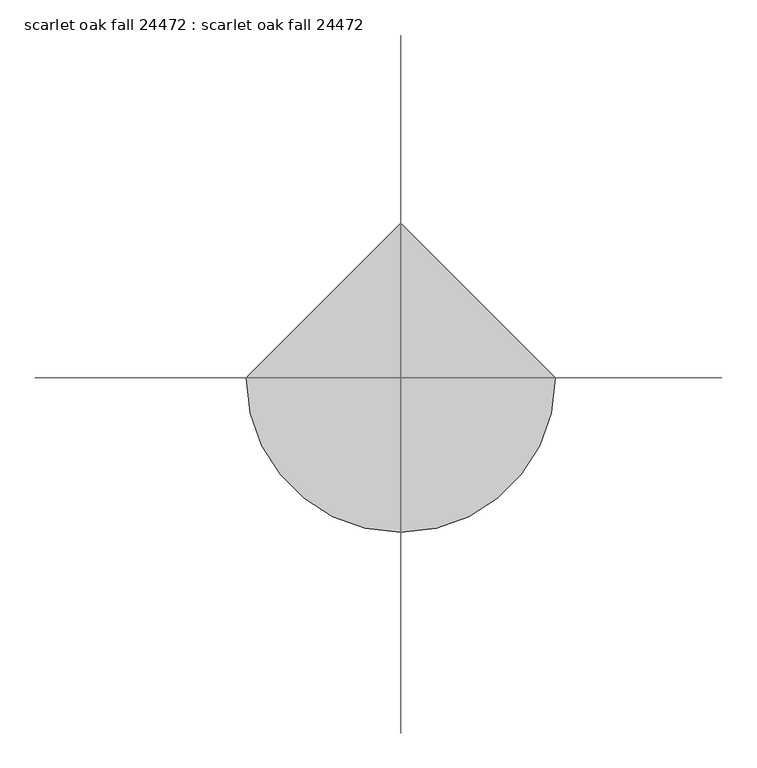
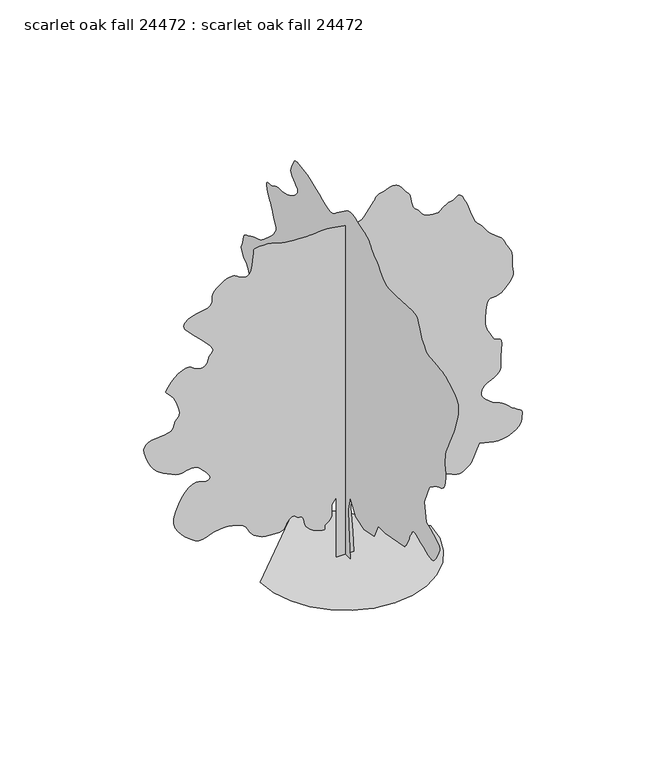
"""IFC4 building model written with IfcOpenShell, lengths in millimetres: proxy geometry, scarlet oak fall 24472 : scarlet oak fall 24472."""

from ifc_helpers import new_model, si_unit, origin, place, context, project, spatial, triangles, source, transform, mapped, element, save


def scarlet_oak_fall_24472_scarlet_oak_fall_24472_7ddbc09d(model_context):
    return source(origin(), model_context, "Body", "Tessellation", [
        triangles([(0.0175265, 310.9036245, 0.0), (0.0175265, -298.2620451, 0.0), (0.0175265, -200.0097575, 1159.3779247), (0.0175265, -180.3587949, 1709.5902706), (0.0175265, -298.2620451, 2220.5035618), (0.0175265, -612.6708881, 1709.5902706), (0.0175265, -1123.5817085, 1552.3870754), (0.0175265, -1713.0954346, 1689.9407433), (0.0175265, -1948.9013901, 2181.2021816), (0.0175265, -2361.5625389, 2181.2021816), (0.0175265, -3501.2886108, 2397.3587551), (0.0175265, -3543.2238419, 2447.9453476), (0.0175265, -3584.1434372, 2498.8747971), (0.0175265, -3622.9800201, 2550.4902512), (0.0175265, -3658.7176643, 2603.1445953), (0.0175265, -3690.3407341, 2657.1703674), (0.0175265, -3716.8074326, 2712.9233597), (0.0175265, -3737.102124, 2770.7082047), (0.0175265, -3756.8125488, 2830.2458496), (0.0175265, -3781.6790543, 2890.7994209), (0.0175265, -3810.8383209, 2952.2166023), (0.0175265, -3843.4264481, 3014.3197884), (0.0175265, -3878.6054054, 3076.9307922), (0.0175265, -3915.4862938, 3139.8972977), (0.0175265, -3953.2560814, 3203.0164101), (0.0175265, -3971.239286, 3223.4125488), (0.0175265, -3996.1057915, 3239.8717186), (0.0175265, -4034.7139, 3248.4060814), (0.0175265, -4093.9466217, 3245.0786682), (0.0175265, -4180.6878387, 3225.9525101), (0.0175265, -4301.7949814, 3187.039769), (0.0175265, -4464.1516411, 3124.4287651), (0.0175265, -4635.5763519, 3050.7434372), (0.0175265, -4781.5502907, 2984.9826256), (0.0175265, -4905.5273163, 2932.6079155), (0.0175265, -5010.9377426, 2899.1561783), (0.0175265, -5101.2345566, 2890.113707), (0.0175265, -5179.8222015, 2910.9670853), (0.0175265, -5250.1801163, 2967.228186), (0.0175265, -5321.172876, 3055.8486488), (0.0175265, -5394.553862, 3163.7225876), (0.0175265, -5463.1339783, 3281.2229736), (0.0175265, -5519.6741318, 3398.7233597), (0.0175265, -5556.9613907, 3506.5970078), (0.0175265, -5567.8072403, 3595.2430504), (0.0175265, -5544.9470078, 3654.9838806), (0.0175265, -5489.0922775, 3699.9671814), (0.0175265, -5408.4727798, 3750.0815643), (0.0175265, -5307.2539581, 3804.513707), (0.0175265, -5189.4995178, 3862.3750008), (0.0175265, -5059.4004822, 3922.8268341), (0.0175265, -4921.0467178, 3984.9805984), (0.0175265, -4778.5783791, 4047.9982635), (0.0175265, -4660.6716225, 4716.1196915), (0.0175265, -4955.4132248, 5403.875386), (0.0175265, -4964.7097504, 5417.0071426), (0.0175265, -4979.1367767, 5433.0346527), (0.0175265, -5003.9015442, 5454.9298279), (0.0175265, -5044.1101364, 5485.5872589), (0.0175265, -5104.9430511, 5527.903862), (0.0175265, -5191.5825302, 5584.850386), (0.0175265, -5309.1334946, 5659.3487457), (0.0175265, -5436.6669891, 5726.8364868), (0.0175265, -5549.7478775, 5770.9308884), (0.0175265, -5648.4011581, 5806.7955597), (0.0175265, -5732.6279938, 5849.5441132), (0.0175265, -5802.4016418, 5914.2884171), (0.0175265, -5857.7482635, 6016.1426651), (0.0175265, -5898.6422791, 6170.2443054), (0.0175265, -5922.3152527, 6321.6030899), (0.0175265, -5929.1223953, 6418.6564682), (0.0175265, -5923.915155, 6481.6735519), (0.0175265, -5911.4694031, 6530.949614), (0.0175265, -5896.6354248, 6586.7537659), (0.0175265, -5884.2152527, 6669.354538), (0.0175265, -5879.0080124, 6799.0722015), (0.0175265, -5880.8369705, 6942.175676), (0.0175265, -5888.8632248, 7060.8701752), (0.0175265, -5906.8464294, 7169.2769302), (0.0175265, -5938.5712372, 7281.4433395), (0.0175265, -5987.8467178, 7411.4917969), (0.0175265, -6058.4336884, 7573.5179535), (0.0175265, -6154.0900589, 7781.5947876), (0.0175265, -6244.9205612, 7969.6821442), (0.0175265, -6305.4738419, 8083.1694031), (0.0175265, -6346.419017, 8153.3494217), (0.0175265, -6378.4484573, 8211.4900589), (0.0175265, -6412.2045364, 8288.8835907), (0.0175265, -6458.3057922, 8416.8234558), (0.0175265, -6527.4701752, 8626.5513519), (0.0175265, -6601.9935333, 8869.1720078), (0.0175265, -6652.1329147, 9078.1127426), (0.0175265, -6670.2940155, 9258.1732635), (0.0175265, -6648.9075302, 9414.1800201), (0.0175265, -6580.4541504, 9550.9338821), (0.0175265, -6457.3407349, 9673.2345566), (0.0175265, -6271.9968155, 9785.9340729), (0.0175265, -6092.164769, 9878.5679535), (0.0175265, -5973.8772217, 9942.3477814), (0.0175265, -5892.0130325, 9984.43591), (0.0175265, -5821.4772217, 10012.1214294), (0.0175265, -5737.1998077, 10032.5690186), (0.0175265, -5614.0858109, 10053.0154449), (0.0175265, -5427.0402512, 10080.7009644), (0.0175265, -5226.405986, 10102.5205627), (0.0175265, -5070.8056, 10110.9526062), (0.0175265, -4947.513707, 10121.4182465), (0.0175265, -4843.8310822, 10149.4339783), (0.0175265, -4747.0061783, 10210.4442078), (0.0175265, -4644.3394798, 10319.9445007), (0.0175265, -4523.1050194, 10493.3501953), (0.0175265, -4417.2379349, 10684.0025116), (0.0175265, -4354.6778, 10837.2152527), (0.0175265, -4313.7837845, 10956.3661194), (0.0175265, -4272.8641891, 11044.9362946), (0.0175265, -4210.3040543, 11106.353476), (0.0175265, -4104.4369698, 11144.0476868), (0.0175265, -3933.5965256, 11161.4710419), (0.0175265, -2990.3674713, 11102.5176636), (0.0175265, -2816.5045372, 11105.5663147), (0.0175265, -2674.9503868, 11105.1593628), (0.0175265, -2554.6812744, 11112.322879), (0.0175265, -2444.7449615, 11138.027124), (0.0175265, -2334.1178478, 11193.3225861), (0.0175265, -2211.8040928, 11289.1574341), (0.0175265, -2066.8032051, 11436.5786682), (0.0175265, -1927.0752514, 11585.474231), (0.0175265, -1822.4043148, 11686.9215271), (0.0175265, -1744.5483112, 11753.6721039), (0.0175265, -1685.2519306, 11798.4275116), (0.0175265, -1636.2706181, 11833.8858124), (0.0175265, -1589.3492088, 11872.7729736), (0.0175265, -1536.2428574, 11927.8405426), (0.0175265, -1485.2548359, 11992.8644806), (0.0175265, -1443.5456085, 12053.4177612), (0.0175265, -1401.1529926, 12109.8573395), (0.0175265, -1348.1024517, 12162.4855225), (0.0175265, -1274.4272976, 12211.7104248), (0.0175265, -1170.1577173, 12257.8366791), (0.0175265, -1025.3294209, 12301.1944977), (0.0175265, -862.7415253, 12348.971814), (0.0175265, -711.1517956, 12401.9057922), (0.0175265, -569.5289721, 12450.7249054), (0.0175265, -436.8469909, 12486.1320465), (0.0175265, -312.0695054, 12498.8580139), (0.0175265, -194.1657283, 12479.604538), (0.0175265, -82.1065163, 12419.1012543), (0.0175265, 507.4081999, 11986.7939209), (0.0175265, 571.2282506, 11928.7044434), (0.0175265, 632.9883253, 11875.7704651), (0.0175265, 700.2449759, 11833.124231), (0.0175265, 780.5673986, 11805.9712372), (0.0175265, 881.5121092, 11799.4437286), (0.0175265, 1010.6431807, 11818.6960419), (0.0175265, 1175.5247589, 11868.8871643), (0.0175265, 1362.6338322, 11943.4105225), (0.0175265, 1551.1170948, 12027.2309875), (0.0175265, 1737.537838, 12112.7780914), (0.0175265, 1918.4594982, 12192.4581116), (0.0175265, 2090.445512, 12258.7517395), (0.0175265, 2250.0539383, 12304.0652527), (0.0175265, 2393.8535912, 12320.8549255), (0.0175265, 2524.6458984, 12330.0241333), (0.0175265, 2646.1466217, 12350.8775116), (0.0175265, 2756.3317566, 12373.4331116), (0.0175265, 2853.0805023, 12387.7578186), (0.0175265, 2934.3860046, 12383.8720093), (0.0175265, 2998.139962, 12351.7914093), (0.0175265, 3042.3105217, 12281.5352325), (0.0175265, 3081.7819496, 12193.2708527), (0.0175265, 3127.0957535, 12111.863031), (0.0175265, 3169.6661201, 12034.5712372), (0.0175265, 3200.9081085, 11958.6502899), (0.0175265, 3212.1856178, 11881.3840759), (0.0175265, 3194.9389961, 11799.9762543), (0.0175265, 3140.5830116, 11711.6862946), (0.0175265, 3057.3979729, 11630.7877441), (0.0175265, 2968.3455597, 11567.4148682), (0.0175265, 2886.8880318, 11512.6519318), (0.0175265, 2826.3850388, 11457.5343658), (0.0175265, 2800.2738419, 11393.1452728), (0.0175265, 2821.9146721, 11310.5445007), (0.0175265, 2904.7694984, 11200.765155), (0.0175265, 3019.1712364, 11091.3927612), (0.0175265, 3127.0448845, 11011.6115845), (0.0175265, 3229.076738, 10954.8173767), (0.0175265, 3325.9522202, 10914.5582062), (0.0175265, 3418.3576263, 10884.2309875), (0.0175265, 3507.0033783, 10857.3826263), (0.0175265, 3592.525193, 10827.4112), (0.0175265, 3677.9455605, 10804.3219116), (0.0175265, 3765.7785713, 10796.7026093), (0.0175265, 3855.9995178, 10795.9654449), (0.0175265, 3948.6333984, 10793.5016418), (0.0175265, 4043.6802132, 10780.7256775), (0.0175265, 4141.139962, 10749.0264496), (0.0175265, 4240.9873558, 10689.8695953), (0.0175265, 4344.1874519, 10637.3169891), (0.0175265, 4445.6350388, 10618.4704651), (0.0175265, 4536.4402519, 10614.0509674), (0.0175265, 4607.6617767, 10604.8306), (0.0175265, 4650.3338814, 10571.5570496), (0.0175265, 4655.540831, 10494.9500977), (0.0175265, 4614.3674721, 10355.8085907), (0.0175265, 4553.5089775, 10209.3779938), (0.0175265, 4502.988224, 10110.7247131), (0.0175265, 4458.6400589, 10040.2394806), (0.0175265, 4416.3743248, 9978.3653503), (0.0175265, 4372.025869, 9905.4918915), (0.0175265, 4321.4798264, 9802.0377411), (0.0175265, 4260.6469116, 9648.393631), (0.0175265, 4196.3595566, 9497.2633209), (0.0175265, 4141.038224, 9401.8104263), (0.0175265, 4098.7472008, 9343.1361008), (0.0175265, 4073.6522209, 9302.3438232), (0.0175265, 4069.8675682, 9260.5353287), (0.0175265, 4091.5336876, 9198.7629364), (0.0175265, 4142.740155, 9098.1789597), (0.0175265, 4233.9008698, 8964.8539581), (0.0175265, 4361.815155, 8823.2998077), (0.0175265, 4510.3796333, 8682.0758698), (0.0175265, 4663.3894798, 8549.7926651), (0.0175265, 4804.7404449, 8435.0357162), (0.0175265, 4918.2277039, 8346.4149628), (0.0175265, 4987.7217178, 8292.4909286), (0.0175265, 5049.4185333, 8258.7592667), (0.0175265, 5142.0524139, 8224.6723938), (0.0175265, 5253.2537659, 8189.9000977), (0.0175265, 5370.6524139, 8154.0860046), (0.0175265, 5481.8537659, 8116.9004837), (0.0175265, 5574.4876465, 8078.0133224), (0.0175265, 5636.1838806, 8037.0425674), (0.0175265, 5687.8475876, 8003.0068542), (0.0175265, 5753.6336884, 7978.9530899), (0.0175265, 5825.9217178, 7955.5853302), (0.0175265, 5897.1941116, 7923.6064682), (0.0175265, 5959.8815643, 7873.7717194), (0.0175265, 6006.3891907, 7796.7589783), (0.0175265, 6029.1982635, 7683.3222977), (0.0175265, 6047.8674728, 7569.3780899), (0.0175265, 6079.9474915, 7488.7835907), (0.0175265, 6114.7709473, 7429.1447891), (0.0175265, 6141.7204651, 7378.0903473), (0.0175265, 6150.0769318, 7323.2774139), (0.0175265, 6129.2235535, 7252.2846542), (0.0175265, 6068.4917953, 7152.7674728), (0.0175265, 5993.1045364, 7059.5493256), (0.0175265, 5932.1448853, 7003.8213318), (0.0175265, 5880.8113907, 6967.6776077), (0.0175265, 5834.2787659, 6933.2349426), (0.0175265, 5787.7711395, 6882.638031), (0.0175265, 5736.437645, 6798.030986), (0.0175265, 5675.4779938, 6661.5055984), (0.0175265, 5609.0314682, 6524.7523178), (0.0175265, 5548.0712357, 6438.5447891), (0.0175265, 5498.1097504, 6383.604538), (0.0175265, 5464.6577225, 6340.6786697), (0.0175265, 5453.2026077, 6290.5642868), (0.0175265, 5469.2295364, 6213.9579163), (0.0175265, 5518.277124, 6091.6566605), (0.0175265, 5583.4283798, 5957.8747101), (0.0175265, 5644.7694031, 5854.0141891), (0.0175265, 5703.392569, 5771.4645767), (0.0175265, 5760.2629349, 5701.6141891), (0.0175265, 5816.4734573, 5635.9048279), (0.0175265, 5873.0136108, 5565.7242279), (0.0175265, 5930.9257736, 5482.4886108), (0.0175265, 5998.1338806, 5400.3959473), (0.0175265, 6076.3407349, 5333.4157333), (0.0175265, 6157.2904449, 5272.6339783), (0.0175265, 6232.753862, 5209.0832062), (0.0175265, 6294.4506775, 5133.8738434), (0.0175265, 6334.1505798, 5038.0139969), (0.0175265, 6343.5994217, 4912.614093), (0.0175265, 6351.5495178, 4814.1384178), (0.0175265, 6380.8355209, 4781.651738), (0.0175265, 6414.2369705, 4780.1024139), (0.0175265, 6434.5822403, 4774.4382248), (0.0175265, 6424.6508698, 4729.5816605), (0.0175265, 6367.3229736, 4610.4810814), (0.0175265, 6245.3519302, 4382.0589775), (0.0175265, 6117.819017, 4125.8490349), (0.0175265, 6040.8312744, 3937.3811783), (0.0175265, 5992.6981659, 3802.5071434), (0.0175265, 5951.8041504, 3707.1809853), (0.0175265, 5896.4575287, 3637.2800194), (0.0175265, 5805.0177612, 3578.7330116), (0.0175265, 5655.8437271, 3517.4428574), (0.0175265, 5483.6059845, 3467.7098465), (0.0175265, 5332.0187256, 3446.8561775), (0.0175265, 5192.8016418, 3445.2559845), (0.0175265, 5057.7244217, 3453.2825294), (0.0175265, 4918.5067566, 3461.2834946), (0.0175265, 4766.9197884, 3459.6833015), (0.0175265, 4594.7076256, 3438.8299232), (0.0175265, 4422.952993, 3420.1610046), (0.0175265, 4274.5661201, 3424.1741318), (0.0175265, 4144.0610046, 3439.8714294), (0.0175265, 4025.9254829, 3456.2544411), (0.0175265, 3914.6735527, 3462.3250008), (0.0175265, 3804.7930504, 3447.0849426), (0.0175265, 3690.7723938, 3399.5361008), (0.0175265, 3581.6540543, 3348.9900581), (0.0175265, 3491.4078186, 3322.5233597), (0.0175265, 3422.1419884, 3305.6831085), (0.0175265, 3375.9139961, 3284.0422783), (0.0175265, 3354.7812744, 3243.1229736), (0.0175265, 3360.8009651, 3168.5484558), (0.0175265, 3396.0307915, 3045.815831), (0.0175265, 3452.8505791, 2915.4374519), (0.0175265, 3521.0243248, 2823.1846527), (0.0175265, 3598.6722015, 2762.7581085), (0.0175265, 3683.8638039, 2727.7567566), (0.0175265, 3774.7195953, 2711.8309845), (0.0175265, 3869.3600395, 2708.6053093), (0.0175265, 3965.8800201, 2711.7548264), (0.0175265, 4339.2598457, 2299.1064674), (0.0175265, 4368.5208504, 2252.6422977), (0.0175265, 4396.5877419, 2205.3220757), (0.0175265, 4422.2672791, 2156.2823364), (0.0175265, 4444.3144798, 2104.6617954), (0.0175265, 4461.5608109, 2049.6073071), (0.0175265, 4472.7877419, 1990.2551159), (0.0175265, 4476.800869, 1925.7468441), (0.0175265, 4476.115155, 1858.4875774), (0.0175265, 4471.314576, 1791.9167862), (0.0175265, 4458.2333977, 1726.7225098), (0.0175265, 4432.8082054, 1663.588282), (0.0175265, 4390.8726837, 1603.2049038), (0.0175265, 4328.3125488, 1546.2580891), (0.0175265, 4240.9873558, 1493.4361679), (0.0175265, 4157.7008698, 1448.5772781), (0.0175265, 4099.153862, 1413.687838), (0.0175265, 4049.1917953, 1386.7054733), (0.0175265, 3991.6610046, 1365.5650486), (0.0175265, 3910.4316605, 1348.2066605), (0.0175265, 3789.3245178, 1332.5653187), (0.0175265, 3612.1850395, 1316.5811199), (0.0175265, 3410.6865829, 1318.8721138), (0.0175265, 3225.0127419, 1354.1629829), (0.0175265, 3051.7084946, 1414.5488319), (0.0175265, 2887.3449806, 1492.1179344), (0.0175265, 2728.4933395, 1578.9707726), (0.0175265, 2571.6738419, 1667.1976547), (0.0175265, 2413.5029732, 1748.8916508), (0.0175265, 2272.4543152, 1823.1968536), (0.0175265, 2163.3739094, 1893.3770176), (0.0175265, 2077.3237839, 1957.7152416), (0.0175265, 2005.3681469, 2014.4892471), (0.0175265, 1938.5687359, 2061.9822784), (0.0175265, 1867.9871429, 2098.4769985), (0.0175265, 1784.687867, 2122.2512741), (0.0175265, 1693.0802319, 2142.3020851), (0.0175265, 1602.8492569, 2167.1661198), (0.0175265, 1512.9611389, 2194.438147), (0.0175265, 1422.387307, 2221.7075581), (0.0175265, 1330.0913418, 2246.5715927), (0.0175265, 1235.0471432, 2266.6224037), (0.0175265, 1136.2233061, 2279.4544693), (0.0175265, 1035.1643583, 2286.1575485), (0.0175265, 934.1027945, 2289.7669212), (0.0175265, 833.0438467, 2290.7981083), (0.0175265, 731.9848263, 2289.7669212), (0.0175265, 630.9258785, 2287.1887356), (0.0175265, 529.864351, 2283.5795082), (0.0175265, 428.8053669, 2279.4544693), (0.0175265, 232.3013002, 1984.6976063), (0.0175265, 192.9998656, 1532.7376934), (284.9321357, 0.0006104, 0.0093596), (-304.5815722, 0.0006104, 0.0093596), (-304.5815722, 0.0004832, 2161.5603573), (-461.7872563, 0.0004832, 1945.4063999), (-461.7872563, 0.0005087, 1709.6004444), (-458.17792, 0.0005087, 1654.888813), (-458.17792, 0.0005087, 1600.3473747), (-465.3965927, 0.0005087, 1546.1514095), (-483.4407675, 0.0005341, 1492.4709652), (-515.9248312, 0.0005341, 1439.4789963), (-566.4555768, 0.0005341, 1387.3429344), (-638.6398699, 0.0005341, 1336.2406757), (-695.1853283, 0.0005341, 1283.1902802), (-710.8266701, 0.0005341, 1229.4514091), (-707.2172974, 0.0005341, 1181.559783), (-706.0133738, 0.0005341, 1146.037896), (-728.8733156, 0.0005341, 1129.4237211), (-797.4482723, 0.0005341, 1138.2476738), (-933.3966602, 0.0005341, 1179.0375532), (-1088.4814528, 0.0005341, 1242.5731373), (-1204.3791023, 0.0005341, 1314.3561104), (-1287.6199516, 0.0005341, 1393.0172974), (-1344.7395756, 0.0005341, 1477.1750965), (-1382.2654827, 0.0005087, 1565.4579346), (-1406.7282337, 0.0005087, 1656.4914768), (-1424.6607147, 0.0005087, 1748.9018246), (-1429.2428478, 0.0005087, 1774.0502895), (-1436.0601643, 0.0005087, 1798.5130405), (-1447.3453766, 0.0005087, 1821.6042183), (-1465.3361389, 0.0005087, 1842.6277897), (-1492.2602222, 0.0005087, 1860.9031277), (-1530.3602222, 0.0005087, 1875.7417568), (-1581.8637646, 0.0005087, 1886.4554924), (-1633.3673069, 0.0005087, 1904.0983109), (-1673.8702126, 0.0005087, 1933.7757145), (-1709.219363, 0.0004832, 1965.8584946), (-1745.2543728, 0.0004832, 1990.7225292), (-1787.8222687, 0.0004832, 1998.7438419), (-1842.7623745, 0.0004832, 1980.2958401), (-1915.9220078, 0.0005087, 1925.7544018), (-1980.257761, 0.0005087, 1849.4451061), (-2016.7524811, 0.0005087, 1774.8530022), (-2043.2776062, 0.0005087, 1706.1053089), (-2077.707336, 0.0005087, 1647.3247398), (-2137.9206665, 0.0005087, 1602.6409847), (-2241.7862743, 0.0005087, 1576.1716702), (-2407.1834461, 0.0005087, 1572.0466312), (-2589.9363899, 0.0005087, 1584.1929829), (-2738.3232628, 0.0005087, 1604.2437939), (-2858.8464294, 0.0005087, 1632.8898651), (-2958.0839767, 0.0005087, 1670.8145851), (-3042.5389961, 0.0005087, 1718.7089001), (-3118.713707, 0.0005087, 1777.2608494), (-3193.211776, 0.0005087, 1847.1541122), (-3256.3817574, 0.0005087, 1923.8062649), (-3301.7205597, 0.0004832, 2000.8063614), (-3340.1507721, 0.0004832, 2076.0843246), (-3382.7214294, 0.0004832, 2147.5827221), (-3440.4048271, 0.0004832, 2213.2367088), (-3524.2247108, 0.0004832, 2270.9860909), (-3645.154248, 0.0004832, 2318.7660233), (-3766.7439194, 0.0004832, 2355.0854633), (-3854.9580116, 0.0004578, 2380.7522106), (-3924.6302124, 0.0004578, 2397.1378384), (-3990.5180511, 0.0004578, 2405.6162453), (-4067.3781853, 0.0004578, 2407.5645275), (-4170.0451744, 0.0004578, 2404.3564384), (-4313.275676, 0.0004578, 2397.3663128), (-4470.7555984, 0.0004578, 2372.5607048), (-4610.7351357, 0.0004832, 2326.4420082), (-4739.6909271, 0.0004832, 2276.1982727), (-4864.1763519, 0.0004832, 2239.0176933), (-4990.7447891, 0.0004832, 2232.0859943), (-5125.8725876, 0.0004832, 2272.5889), (-5276.1389969, 0.0004578, 2377.7169308), (-5433.3648651, 0.0004578, 2518.3058784), (-5578.5257721, 0.0004578, 2657.8560814), (-5702.0461395, 0.0004324, 2802.5853287), (-5794.2736496, 0.0004324, 2958.6429543), (-5845.6071442, 0.0004324, 3132.226545), (-5846.4198853, 0.0004069, 3329.5336876), (-5787.0601364, 0.0004069, 3556.7366798), (-5687.7208511, 0.0003815, 3785.8956573), (-5577.0276077, 0.0003815, 3982.4153481), (-5458.1046341, 0.0003561, 4142.4861008), (-5334.0255798, 0.0003561, 4262.3232628), (-5207.8635132, 0.0003561, 4338.1677612), (-5082.7432434, 0.0003561, 4366.2602325), (-4961.7378387, 0.0003561, 4342.765155), (-4847.6154442, 0.0003561, 4303.2428581), (-4746.5742279, 0.0003561, 4286.3770271), (-4666.8183403, 0.0003561, 4293.2606186), (-4616.6277992, 0.0003561, 4324.8833977), (-4604.2582054, 0.0003561, 4382.2874519), (-4637.9384171, 0.0003561, 4466.5139969), (-4725.9240349, 0.0003306, 4578.5786682), (-4828.540155, 0.0003306, 4690.9738426), (-4906.7470093, 0.0003306, 4777.5877419), (-4969.8146713, 0.0003306, 4841.5195953), (-5027.0414108, 0.0003306, 4885.8680511), (-5087.7220093, 0.0003306, 4913.7064682), (-5161.1024139, 0.0003052, 4928.1590744), (-5256.5047302, 0.0003052, 4932.2739395), (-5354.3458511, 0.0003306, 4923.0535721), (-5435.3717194, 0.0003306, 4901.7938232), (-5509.1584946, 0.0003306, 4878.1464294), (-5585.3584946, 0.0003306, 4861.6872597), (-5673.5728775, 0.0003306, 4862.0936302), (-5783.4533798, 0.0003306, 4888.9666992), (-5924.6261581, 0.0003052, 4951.9332047), (-6074.4356186, 0.0003052, 5027.2698853), (-6206.363031, 0.0003052, 5092.6240356), (-6324.2192093, 0.0003052, 5159.730986), (-6431.7376465, 0.0003052, 5240.2231659), (-6532.7529922, 0.0003052, 5345.7859085), (-6631.0004837, 0.0002798, 5488.1528), (-6730.2891907, 0.0002798, 5679.0085922), (-6812.3818542, 0.0002543, 5877.0523178), (-6857.6953674, 0.0002543, 6036.2594604), (-6867.9569504, 0.0002543, 6161.1006775), (-6844.8682434, 0.0002289, 6256.0204651), (-6790.157048, 0.0002289, 6325.5144791), (-6705.5494217, 0.0002289, 6374.0283783), (-6592.7225876, 0.0002289, 6406.0578186), (-6459.5249039, 0.0002289, 6424.4473938), (-6318.7834946, 0.0002289, 6435.2932434), (-6179.7187271, 0.0002289, 6447.8157349), (-6051.677124, 0.0002289, 6471.3613907), (-5943.9302124, 0.0002289, 6515.201738), (-5865.7239395, 0.0002289, 6588.5821426), (-5826.3536682, 0.0002035, 6700.8252914), (-5797.2705597, 0.0002035, 6809.207048), (-5752.3384186, 0.0002035, 6879.7934372), (-5704.6878387, 0.0002035, 6934.9115845), (-5667.3244217, 0.0002035, 6996.8874527), (-5653.3543442, 0.000178, 7088.0987457), (-5675.8082062, 0.000178, 7230.8720078), (-5747.7660233, 0.000178, 7447.5343643), (-5849.6708496, 0.0001526, 7660.9451752), (-5947.1305984, 0.0001526, 7795.2858124), (-6030.8237457, 0.0001526, 7874.990831), (-6091.5043442, 0.0001272, 7924.4192093), (-6119.8508698, 0.0001272, 7968.0055023), (-6106.6173752, 0.0001272, 8030.1848465), (-6042.5079163, 0.0001272, 8135.3156387), (-5939.1805023, 0.0001272, 8266.5064682), (-5819.6738434, 0.0001017, 8386.0137085), (-5691.911293, 0.0001017, 8486.9528961), (-5563.7941132, 0.0001017, 8562.4674728), (-5443.2712372, 0.0001017, 8605.6473953), (-5338.1910233, 0.0001017, 8609.6605225), (-5256.5047302, 0.0001017, 8567.6235535), (-5176.4183395, 0.0001017, 8504.9361008), (-5077.7650589, 0.0001017, 8456.015831), (-4970.8564682, 0.0001017, 8427.3646729), (-4866.0050194, 0.0001017, 8425.5357147), (-4773.5490349, 0.0001017, 8457.0570465), (-4703.7753868, 0.0001017, 8528.4311783), (-4666.9962364, 0.0001017, 8646.2111984), (-4633.2904449, 0.0001017, 8758.5043442), (-4580.3567574, 7.63e-05, 8825.0776062), (-4529.8360039, 7.63e-05, 8869.9853302), (-4503.3693054, 7.63e-05, 8917.3051163), (-4522.6224907, 7.63e-05, 8991.0924728), (-4609.2366806, 7.63e-05, 9115.425), (-4784.902993, 5.09e-05, 9314.3326263), (-5005.1718155, 5.09e-05, 9539.0212372), (-5202.0725876, 2.54e-05, 9728.3021255), (-5361.8639969, 2.54e-05, 9887.6871643), (-5470.753862, 2.54e-05, 10022.6626465), (-5515.0511581, 0.0, 10138.7404449), (-5480.9642853, 0.0, 10241.4074341), (-5354.7522217, 0.0, 10336.1493256), (-5186.4258682, 0.0, 10409.1483582), (-5035.6519318, 0.0, 10450.8562775), (-4903.089093, 0.0, 10473.3095581), (-4789.4242287, -2.54e-05, 10488.5493256), (-4695.3424713, -2.54e-05, 10508.5899628), (-4621.5554054, -2.54e-05, 10545.4958496), (-4568.7234558, -2.54e-05, 10611.2569519), (-4542.3837845, -2.54e-05, 10689.0568542), (-4538.3706573, -2.54e-05, 10757.2306), (-4542.9424713, -2.54e-05, 10820.603476), (-4542.3837845, -2.54e-05, 10883.9763519), (-4522.9018341, -5.09e-05, 10952.1500977), (-4470.7555984, -5.09e-05, 11029.95), (-4372.2290543, -5.09e-05, 11122.1780914), (-4251.6300201, -5.09e-05, 11213.4399628), (-4141.3431473, -5.09e-05, 11284.4333038), (-4039.6667953, -7.63e-05, 11334.0895752), (-3944.8487457, -7.63e-05, 11361.4204651), (-3855.1867767, -7.63e-05, 11365.3830139), (-3768.9536682, -7.63e-05, 11344.909845), (-3684.4733597, -5.09e-05, 11299.0382263), (-3597.3766411, -5.09e-05, 11242.9544403), (-3507.5623558, -5.09e-05, 11199.2408295), (-3419.4497108, -5.09e-05, 11177.8549255), (-3337.5093636, -5.09e-05, 11188.8019318), (-3266.2369698, -5.09e-05, 11242.0149628), (-3210.1028961, -7.63e-05, 11347.5015472), (-3173.5522202, -7.63e-05, 11515.1924744), (-3151.7337845, -7.63e-05, 11695.2524139), (-3136.0873558, -0.0001017, 11834.3939209), (-3125.5970078, -0.0001017, 11937.4666992), (-3119.2471046, -0.0001017, 12009.2472015), (-3115.9705605, -0.0001017, 12054.5607147), (-3114.776738, -0.0001017, 12078.2336884), (-3114.5988419, -0.0001017, 12085.0414124), (-3088.7669884, -0.0001017, 12089.0539581), (-3018.5869698, -0.0001017, 12097.8929535), (-2915.0563705, -0.0001017, 12106.7075317), (-2789.1995178, -0.0001017, 12110.7200775), (-2651.988707, -0.0001017, 12105.1064667), (-2514.4299522, -0.0001017, 12085.0414124), (-2387.5340641, -0.0001017, 12045.7472992), (-2271.1766315, -0.0001017, 12002.0336884), (-2154.476342, -0.0001017, 11970.3600403), (-2032.2769695, -0.0001017, 11948.286969), (-1899.419672, -0.0001017, 11933.4541534), (-1750.7534557, -0.0001017, 11923.4466248), (-1581.1170078, -0.0001017, 11915.8261597), (-1385.3567184, -0.0001017, 11908.2056946), (-1196.4162163, -0.0001017, 11907.1139008), (-1040.8158302, -0.0001017, 11916.3342682), (-903.7777559, -0.0001017, 11929.3392883), (-770.5217182, -0.0001017, 11939.6002899), (-626.2675146, -0.0001017, 11940.5653473), (-456.2297467, -0.0001017, 11925.7325317), (-245.6314641, -0.0001017, 11888.5464294), (-32.7413631, -0.0001017, 11844.3247101), (138.8999065, -0.0001017, 11813.8451752), (276.1665915, -0.0001017, 11798.8333008), (385.9352365, -0.0001017, 11800.9924713), (475.0790686, -0.0001017, 11822.1004852), (550.4713417, -0.0001017, 11863.8072418), (618.9904152, -0.0001017, 11927.8405426), (913.7472782, -0.0001272, 12301.1944977), (957.9762646, -0.0001272, 12358.7770294), (993.267061, -0.0001272, 12412.929538), (1025.1186052, -0.0001272, 12462.586972), (1059.035285, -0.0001272, 12506.7575317), (1100.5134218, -0.0001272, 12544.3994202), (1155.0548601, -0.0001272, 12574.4731659), (1228.1561394, -0.0001272, 12595.9625519), (1317.7570656, -0.0001526, 12620.5994202), (1415.6080696, -0.0001526, 12653.4927612), (1517.9269695, -0.0001526, 12683.6176666), (1620.9366703, -0.0001526, 12700.0003876), (1720.8500484, -0.0001526, 12691.6439209), (1813.8876835, -0.0001526, 12647.5245209), (1896.2726257, -0.0001272, 12556.6684387), (1969.4296429, -0.0001272, 12453.0363922), (2036.4018631, -0.0001272, 12372.4168945), (2095.8124809, -0.0001272, 12306.5802155), (2146.2848362, -0.0001272, 12247.2966248), (2186.4447395, -0.0001272, 12186.2852325), (2214.9181469, -0.0001017, 12115.2918915), (2230.3283981, -0.0001017, 12026.0880341), (2241.0421337, -0.0001017, 11933.6320496), (2255.8807629, -0.0001017, 11856.6437256), (2274.1561008, -0.0001017, 11792.534848), (2295.1796722, -7.63e-05, 11738.736969), (2318.2682339, -7.63e-05, 11692.6618744), (2342.7309849, -7.63e-05, 11651.7678589), (2367.882066, -7.63e-05, 11613.4388031), (2393.3175774, -7.63e-05, 11596.1921814), (2419.7868919, -7.63e-05, 11576.5329163), (2448.3162552, -7.63e-05, 11552.0727814), (2479.9416504, -7.63e-05, 11520.3991333), (2515.6897591, -7.63e-05, 11479.0981659), (2556.5863907, -7.63e-05, 11425.7583984), (2603.677993, -7.63e-05, 11357.9916046), (2673.4772209, -5.09e-05, 11293.5769318), (2772.1307922, -5.09e-05, 11249.4831116), (2885.2113899, -5.09e-05, 11221.8475891), (2998.2922783, -5.09e-05, 11206.9624512), (3096.9458496, -5.09e-05, 11200.9942108), (3166.7450775, -5.09e-05, 11200.2070496), (3193.211776, -5.09e-05, 11200.7907349), (3206.7754829, -5.09e-05, 11214.9387085), (3244.088031, -5.09e-05, 11251.4132263), (3299.9427612, -5.09e-05, 11301.3241333), (3369.2085915, -7.63e-05, 11355.6801178), (3446.7038612, -7.63e-05, 11405.5910248), (3527.3236496, -7.63e-05, 11442.0911224), (3605.8604256, -7.63e-05, 11456.2390961), (3676.2692093, -7.63e-05, 11473.4857178), (3738.4229736, -7.63e-05, 11512.372879), (3796.1316605, -7.63e-05, 11553.6726837), (3853.1293442, -7.63e-05, 11578.1583984), (3913.225676, -7.63e-05, 11566.5253876), (3980.2055992, -7.63e-05, 11499.545755), (4057.8278961, -7.63e-05, 11357.9916046), (4130.929248, -5.09e-05, 11191.6726868), (4185.462838, -5.09e-05, 11057.3320496), (4226.9411201, -5.09e-05, 10946.0027985), (4260.8500969, -2.54e-05, 10848.7971039), (4292.7016411, -2.54e-05, 10756.7224915), (4328.0076256, -2.54e-05, 10660.8888062), (4372.2290543, -2.54e-05, 10552.3035736), (4417.6695946, 0.0, 10457.0279938), (4456.5570465, 0.0, 10396.4747131), (4494.4285721, 0.0, 10354.8435333), (4536.7704643, 0.0, 10316.2865845), (4589.0690163, 0.0, 10265.0036682), (4656.8361008, 0.0, 10185.1969116), (4745.5838814, 0.0, 10061.0416992), (4854.829248, 2.54e-05, 9922.8664124), (4974.7422775, 2.54e-05, 9807.3722992), (5096.7133209, 2.54e-05, 9708.362645), (5212.1562744, 5.09e-05, 9619.6913132), (5312.4611984, 5.09e-05, 9535.1348465), (5389.067569, 5.09e-05, 9448.4953674), (5433.3648651, 5.09e-05, 9353.6267395), (5468.1377426, 5.09e-05, 9260.5864883), (5516.6516418, 7.63e-05, 9177.1723938), (5571.0332062, 7.63e-05, 9093.7588806), (5623.3317581, 7.63e-05, 9000.7186295), (5665.6733597, 7.63e-05, 8888.4510635), (5690.1334946, 0.0001017, 8747.2777039), (5688.812645, 0.0001017, 8567.6235535), (5686.1203674, 0.0001017, 8394.9544418), (5700.9537643, 0.0001272, 8269.0208496), (5717.1591705, 0.0001272, 8171.6372589), (5718.6067566, 0.0001272, 8084.540831), (5689.0922791, 0.0001272, 7989.5704651), (5612.510907, 0.0001526, 7868.4377426), (5472.6589783, 0.0001526, 7702.9821442), (5306.6952713, 0.0001526, 7564.069693), (5162.7278961, 0.0001526, 7508.3167007), (5041.0870651, 0.0001526, 7496.2261597), (4942.1541504, 0.0001526, 7488.2760635), (4866.2337845, 0.000178, 7444.8926651), (4813.7064674, 0.000178, 7326.6045364), (4784.8774132, 0.000178, 7093.839093), (4774.1080124, 0.0002035, 6836.2577225), (4775.7334946, 0.0002035, 6654.9780899), (4790.0337845, 0.0002289, 6527.6986496), (4817.4402512, 0.0002289, 6432.0166992), (4858.2328194, 0.0002289, 6345.6312744), (4912.7664093, 0.0002289, 6246.1652527), (4981.3971039, 0.0002543, 6111.316507), (5059.7056961, 0.0002543, 5994.0445953), (5138.7247101, 0.0002543, 5940.7048279), (5211.8772217, 0.0002543, 5918.9875488), (5272.6589767, 0.0002543, 5896.5848465), (5314.5436295, 0.0002543, 5841.1876465), (5330.9775101, 0.0002798, 5720.4612946), (5315.4581085, 0.0002798, 5502.1484573), (5294.3762558, 0.0003052, 5261.4579163), (5291.1502899, 0.0003052, 5085.4105225), (5294.8332047, 0.0003052, 4959.1978775), (5294.3762558, 0.0003306, 4868.0624519), (5278.7806961, 0.0003306, 4797.1964287), (5237.0739395, 0.0003306, 4731.8169891), (5158.2578201, 0.0003306, 4657.1663132), (5063.0328186, 0.0003306, 4587.1639), (4978.8065643, 0.0003306, 4539.8438232), (4904.5622589, 0.0003306, 4506.6205605), (4839.2589775, 0.0003561, 4478.8838814), (4781.8549232, 0.0003561, 4448.0735527), (4731.3344604, 0.0003561, 4405.554055), (4686.6302124, 0.0003561, 4342.765155), (4651.1210426, 0.0003561, 4270.0704643), (4631.0551163, 0.0003561, 4201.4903481), (4629.9121628, 0.0003561, 4133.951738), (4651.1210426, 0.0003815, 4064.3304062), (4698.0856178, 0.0003815, 3989.5779922), (4774.2856178, 0.0003815, 3906.5455605), (4883.1501938, 0.0003815, 3812.2100395), (4998.5169891, 0.0003815, 3729.5328186), (5096.3831085, 0.0003815, 3675.3800194), (5183.2254822, 0.0004069, 3637.4070465), (5265.6233597, 0.0004069, 3603.2187263), (5350.0530899, 0.0004069, 3560.4195946), (5443.0933411, 0.0004069, 3496.6403481), (5551.2466232, 0.0004069, 3399.5361008), (5666.0797302, 0.0004069, 3299.2314674), (5771.9471054, 0.0004069, 3227.4509651), (5864.7583008, 0.0004324, 3174.212645), (5940.3746155, 0.0004324, 3129.5848457), (5994.6794403, 0.0004324, 3083.5856186), (6023.5596542, 0.0004324, 3026.2324333), (6022.8736496, 0.0004324, 2947.5686302), (6011.5958496, 0.0004324, 2858.2621628), (6004.7631271, 0.0004578, 2774.4419884), (5992.4441116, 0.0004578, 2694.4067574), (5964.6568542, 0.0004578, 2616.4539574), (5911.4438232, 0.0004578, 2538.8165451), (5822.8230698, 0.0004578, 2459.8123558), (5688.812645, 0.0004578, 2377.7169308), (5528.7927612, 0.0004832, 2311.2603767), (5368.797876, 0.0004832, 2276.7722202), (5208.7779922, 0.0004832, 2268.9237167), (5048.7581085, 0.0004832, 2282.3856857), (4888.7638046, 0.0004832, 2311.8318535), (4728.7436302, 0.0004832, 2351.9359463), (4568.7234558, 0.0004578, 2397.3663128), (4293.6161201, 0.0005087, 1788.2032047), (4226.2045372, 0.0005087, 1729.7654926), (4158.4118729, 0.0005087, 1674.4239578), (4089.9587837, 0.0005087, 1625.269836), (4020.4644791, 0.0005087, 1585.394363), (3949.5984558, 0.0005087, 1557.8963322), (3877.0052124, 0.0005087, 1545.8669792), (3802.3548271, 0.0005087, 1552.3972492), (3741.5216217, 0.0005087, 1567.2334076), (3703.0152512, 0.0005087, 1579.6666603), (3675.5326263, 0.0005087, 1592.1000584), (3647.6942093, 0.0005087, 1606.9360714), (3608.1463326, 0.0005087, 1626.5880695), (3545.5861977, 0.0005087, 1653.456197), (3448.6598465, 0.0005087, 1689.9509171), (3322.3963326, 0.0005087, 1742.9430313), (3184.4489388, 0.0005087, 1813.1231953), (3042.3613907, 0.0005087, 1893.6158112), (2903.7279922, 0.0004832, 1977.5449905), (2776.0677612, 0.0004832, 2058.0376064), (2667.0, 0.0004832, 2128.2177704), (2584.0437263, 0.0004832, 2181.2123554), (2513.8000488, 0.0004832, 2227.9026741), (2438.4075577, 0.0004832, 2282.8427799), (2358.7151836, 0.0004832, 2344.6613903), (2275.5885715, 0.0004578, 2411.9764675), (2189.8814484, 0.0004578, 2483.4164383), (2102.4571335, 0.0004578, 2557.602317), (2014.1742954, 0.0004578, 2633.1671814), (1994.5222973, 0.0004324, 2927.9343636), (1601.5132919, 0.0004324, 2967.228186), (894.0952801, 0.0004324, 2908.2748077), (422.4858398, 0.0004578, 2652.8267372), (225.9802471, 0.0004832, 2181.2123554), (186.6795937, 0.0005087, 1630.9975388), (245.6304467, 0.0005595, 727.0775677), (-2901.5944016, 0.0, 0.0227886), (-2824.8865837, -664.8552029, 0.0227886), (-2606.4211395, -1275.4204056, 0.0227886), (-2263.6988903, -1814.1975483, 0.0227886), (-1814.1975483, -2263.6988903, 0.0227886), (-1275.4204056, -2606.4211395, 0.0227886), (-664.8552029, -2824.8865837, 0.0227886), (0.0001268, -2901.5944016, 0.0227886), (664.8552029, -2824.8865837, 0.0227886), (1275.4204056, -2606.4211395, 0.0227886), (1814.1975483, -2263.6988903, 0.0227886), (2263.6988903, -1814.1975483, 0.0227886), (2606.4211395, -1275.4204056, 0.0227886), (2824.8865837, -664.8552029, 0.0227886), (2901.5944016, 0.0002543, 0.0227886), (-0.0003805, 2901.5944016, 0.0227886)], [[1, 2, 3], [368, 1, 3], [368, 3, 4], [367, 368, 4], [367, 4, 5], [277, 278, 279], [366, 367, 5], [276, 277, 279], [276, 279, 280], [7, 8, 9], [6, 7, 9], [5, 6, 9], [315, 316, 317], [201, 202, 203], [200, 201, 203], [200, 203, 204], [199, 200, 204], [199, 204, 205], [198, 199, 205], [198, 205, 206], [198, 206, 207], [197, 198, 207], [197, 207, 208], [275, 276, 280], [196, 197, 208], [195, 196, 208], [194, 195, 208], [194, 208, 209], [193, 194, 209], [192, 193, 209], [192, 209, 210], [191, 192, 210], [191, 210, 211], [191, 211, 212], [190, 191, 212], [190, 212, 213], [190, 213, 214], [189, 190, 214], [189, 214, 215], [188, 189, 215], [187, 188, 215], [186, 187, 215], [10, 11, 12], [314, 315, 317], [10, 12, 13], [10, 13, 14], [10, 14, 15], [10, 15, 16], [10, 16, 17], [10, 17, 18], [10, 18, 19], [10, 19, 20], [10, 20, 21], [10, 21, 22], [185, 186, 215], [185, 215, 216], [275, 280, 281], [10, 22, 23], [167, 168, 169], [166, 167, 169], [165, 166, 169], [165, 169, 170], [164, 165, 170], [164, 170, 171], [163, 164, 171], [163, 171, 172], [163, 172, 173], [163, 173, 174], [163, 174, 175], [163, 175, 176], [163, 176, 177], [163, 177, 178], [163, 178, 179], [163, 179, 180], [162, 163, 180], [161, 162, 180], [160, 161, 180], [159, 160, 180], [159, 180, 181], [158, 159, 181], [157, 158, 181], [156, 157, 181], [156, 181, 182], [155, 156, 182], [154, 155, 182], [154, 182, 183], [9, 10, 23], [9, 23, 24], [9, 24, 25], [45, 46, 47], [44, 45, 47], [44, 47, 48], [43, 44, 48], [43, 48, 49], [42, 43, 49], [42, 49, 50], [41, 42, 50], [40, 41, 50], [40, 50, 51], [39, 40, 51], [38, 39, 51], [37, 38, 51], [36, 37, 51], [35, 36, 51], [34, 35, 51], [33, 34, 51], [33, 51, 52], [32, 33, 52], [32, 52, 53], [31, 32, 53], [30, 31, 53], [29, 30, 53], [28, 29, 53], [28, 53, 54], [27, 28, 54], [26, 27, 54], [5, 9, 25], [5, 25, 26], [5, 26, 54], [5, 54, 55], [366, 5, 55], [365, 366, 55], [364, 365, 55], [363, 364, 55], [362, 363, 55], [361, 362, 55], [361, 55, 56], [153, 154, 183], [153, 183, 184], [313, 314, 317], [360, 361, 56], [184, 185, 216], [153, 184, 216], [152, 153, 216], [152, 216, 217], [243, 244, 245], [242, 243, 245], [242, 245, 246], [241, 242, 246], [241, 246, 247], [241, 247, 248], [240, 241, 248], [240, 248, 249], [240, 249, 250], [239, 240, 250], [239, 250, 251], [238, 239, 251], [237, 238, 251], [236, 237, 251], [235, 236, 251], [234, 235, 251], [233, 234, 251], [232, 233, 251], [231, 232, 251], [230, 231, 251], [229, 230, 251], [228, 229, 251], [228, 251, 252], [227, 228, 252], [226, 227, 252], [226, 252, 253], [226, 253, 254], [226, 254, 255], [226, 255, 256], [226, 256, 257], [225, 226, 257], [224, 225, 257], [223, 224, 257], [222, 223, 257], [222, 257, 258], [221, 222, 258], [220, 221, 258], [115, 116, 117], [114, 115, 117], [114, 117, 118], [113, 114, 118], [113, 118, 119], [112, 113, 119], [111, 112, 119], [110, 111, 119], [152, 217, 218], [313, 317, 318], [313, 318, 319], [313, 319, 320], [313, 320, 321], [313, 321, 322], [313, 322, 323], [313, 323, 324], [313, 324, 325], [313, 325, 326], [313, 326, 327], [313, 327, 328], [313, 328, 329], [313, 329, 330], [313, 330, 331], [313, 331, 332], [313, 332, 333], [313, 333, 334], [313, 334, 335], [313, 335, 336], [313, 336, 337], [313, 337, 338], [313, 338, 339], [313, 339, 340], [313, 340, 341], [312, 313, 341], [312, 341, 342], [312, 342, 343], [311, 312, 343], [311, 343, 344], [311, 344, 345], [310, 311, 345], [310, 345, 346], [310, 346, 347], [310, 347, 348], [309, 310, 348], [309, 348, 349], [309, 349, 350], [308, 309, 350], [308, 350, 351], [307, 308, 351], [307, 351, 352], [307, 352, 353], [307, 353, 354], [307, 354, 355], [307, 355, 356], [307, 356, 357], [307, 357, 358], [306, 307, 358], [306, 358, 359], [306, 359, 360], [306, 360, 56], [305, 306, 56], [305, 56, 57], [304, 305, 57], [303, 304, 57], [302, 303, 57], [301, 302, 57], [301, 57, 58], [301, 58, 59], [110, 119, 120], [109, 110, 120], [109, 120, 121], [301, 59, 60], [300, 301, 60], [300, 60, 61], [151, 152, 218], [109, 121, 122], [300, 61, 62], [145, 146, 147], [144, 145, 147], [143, 144, 147], [143, 147, 148], [142, 143, 148], [141, 142, 148], [140, 141, 148], [140, 148, 149], [139, 140, 149], [138, 139, 149], [137, 138, 149], [136, 137, 149], [135, 136, 149], [134, 135, 149], [133, 134, 149], [132, 133, 149], [132, 149, 150], [131, 132, 150], [130, 131, 150], [129, 130, 150], [128, 129, 150], [127, 128, 150], [126, 127, 150], [126, 150, 151], [126, 151, 218], [125, 126, 218], [124, 125, 218], [123, 124, 218], [123, 218, 219], [122, 123, 219], [109, 122, 219], [108, 109, 219], [108, 219, 220], [108, 220, 258], [108, 258, 259], [108, 259, 260], [108, 260, 261], [108, 261, 262], [107, 108, 262], [107, 262, 263], [107, 263, 264], [106, 107, 264], [106, 264, 265], [106, 265, 266], [106, 266, 267], [106, 267, 268], [105, 106, 268], [104, 105, 268], [103, 104, 268], [102, 103, 268], [101, 102, 268], [100, 101, 268], [99, 100, 268], [98, 99, 268], [97, 98, 268], [96, 97, 268], [95, 96, 268], [94, 95, 268], [93, 94, 268], [92, 93, 268], [91, 92, 268], [90, 91, 268], [89, 90, 268], [88, 89, 268], [87, 88, 268], [86, 87, 268], [85, 86, 268], [84, 85, 268], [83, 84, 268], [82, 83, 268], [81, 82, 268], [80, 81, 268], [79, 80, 268], [78, 79, 268], [77, 78, 268], [76, 77, 268], [75, 76, 268], [74, 75, 268], [73, 74, 268], [72, 73, 268], [71, 72, 268], [70, 71, 268], [69, 70, 268], [68, 69, 268], [67, 68, 268], [66, 67, 268], [65, 66, 268], [64, 65, 268], [63, 64, 268], [62, 63, 268], [300, 62, 268], [299, 300, 268], [298, 299, 268], [297, 298, 268], [296, 297, 268], [295, 296, 268], [294, 295, 268], [293, 294, 268], [292, 293, 268], [291, 292, 268], [290, 291, 268], [289, 290, 268], [288, 289, 268], [287, 288, 268], [286, 287, 268], [285, 286, 268], [284, 285, 268], [283, 284, 268], [282, 283, 268], [281, 282, 268], [275, 281, 268], [275, 268, 269], [274, 275, 269], [274, 269, 270], [274, 270, 271], [273, 274, 271], [272, 273, 271], [802, 369, 370], [802, 370, 371], [801, 802, 371], [800, 801, 371], [575, 576, 577], [799, 800, 371], [574, 575, 577], [383, 384, 385], [383, 385, 386], [382, 383, 386], [382, 386, 387], [381, 382, 387], [381, 387, 388], [794, 795, 796], [510, 511, 512], [574, 577, 578], [573, 574, 578], [572, 573, 578], [572, 578, 579], [571, 572, 579], [571, 579, 580], [570, 571, 580], [570, 580, 581], [570, 581, 582], [569, 570, 582], [569, 582, 583], [569, 583, 584], [568, 569, 584], [568, 584, 585], [509, 510, 512], [509, 512, 513], [508, 509, 513], [508, 513, 514], [508, 514, 515], [507, 508, 515], [507, 515, 516], [507, 516, 517], [507, 517, 518], [507, 518, 519], [507, 519, 520], [507, 520, 521], [507, 521, 522], [506, 507, 522], [506, 522, 523], [505, 506, 523], [505, 523, 524], [504, 505, 524], [568, 585, 586], [504, 524, 525], [538, 539, 540], [538, 540, 541], [537, 538, 541], [537, 541, 542], [536, 537, 542], [536, 542, 543], [536, 543, 544], [535, 536, 544], [535, 544, 545], [535, 545, 546], [534, 535, 546], [534, 546, 547], [533, 534, 547], [533, 547, 548], [381, 388, 389], [380, 381, 389], [380, 389, 390], [380, 390, 391], [380, 391, 392], [380, 392, 393], [379, 380, 393], [378, 379, 393], [377, 378, 393], [376, 377, 393], [375, 376, 393], [374, 375, 393], [373, 374, 393], [372, 373, 393], [372, 393, 394], [372, 394, 395], [372, 395, 396], [372, 396, 397], [372, 397, 398], [371, 372, 398], [371, 398, 399], [532, 533, 548], [371, 399, 400], [567, 568, 586], [567, 586, 587], [657, 658, 659], [657, 659, 660], [656, 657, 660], [656, 660, 661], [655, 656, 661], [655, 661, 662], [654, 655, 662], [654, 662, 663], [653, 654, 663], [652, 653, 663], [651, 652, 663], [650, 651, 663], [649, 650, 663], [649, 663, 664], [648, 649, 664], [647, 648, 664], [647, 664, 665], [647, 665, 666], [647, 666, 667], [647, 667, 668], [647, 668, 669], [793, 794, 796], [713, 714, 715], [713, 715, 716], [712, 713, 716], [712, 716, 717], [711, 712, 717], [646, 647, 669], [711, 717, 718], [567, 587, 588], [645, 646, 669], [645, 669, 670], [750, 751, 752], [749, 750, 752], [748, 749, 752], [748, 752, 753], [747, 748, 753], [747, 753, 754], [747, 754, 755], [747, 755, 756], [747, 756, 757], [747, 757, 758], [747, 758, 759], [747, 759, 760], [746, 747, 760], [746, 760, 761], [746, 761, 762], [745, 746, 762], [745, 762, 763], [745, 763, 764], [744, 745, 764], [743, 744, 764], [743, 764, 765], [742, 743, 765], [741, 742, 765], [741, 765, 766], [740, 741, 766], [739, 740, 766], [738, 739, 766], [737, 738, 766], [736, 737, 766], [735, 736, 766], [644, 645, 670], [567, 588, 589], [792, 793, 796], [371, 400, 401], [371, 401, 402], [371, 402, 403], [371, 403, 404], [371, 404, 405], [799, 371, 405], [799, 405, 406], [766, 767, 768], [488, 489, 490], [488, 490, 491], [487, 488, 491], [487, 491, 492], [486, 487, 492], [486, 492, 493], [485, 486, 493], [485, 493, 494], [485, 494, 495], [484, 485, 495], [483, 484, 495], [483, 495, 496], [482, 483, 496], [481, 482, 496], [480, 481, 496], [479, 480, 496], [479, 496, 497], [478, 479, 497], [477, 478, 497], [476, 477, 497], [475, 476, 497], [474, 475, 497], [473, 474, 497], [472, 473, 497], [471, 472, 497], [471, 497, 498], [470, 471, 498], [469, 470, 498], [469, 498, 499], [468, 469, 499], [468, 499, 500], [468, 500, 501], [468, 501, 502], [468, 502, 503], [467, 468, 503], [466, 467, 503], [466, 503, 504], [466, 504, 525], [465, 466, 525], [465, 525, 526], [464, 465, 526], [463, 464, 526], [735, 766, 768], [735, 768, 769], [735, 769, 770], [735, 770, 771], [735, 771, 772], [735, 772, 773], [735, 773, 774], [735, 774, 775], [735, 775, 776], [735, 776, 777], [735, 777, 778], [735, 778, 779], [735, 779, 780], [735, 780, 781], [735, 781, 782], [735, 782, 783], [735, 783, 784], [735, 784, 785], [735, 785, 786], [735, 786, 787], [735, 787, 788], [735, 788, 789], [735, 789, 790], [735, 790, 791], [735, 791, 792], [735, 792, 796], [734, 735, 796], [733, 734, 796], [732, 733, 796], [731, 732, 796], [731, 796, 797], [730, 731, 797], [567, 589, 590], [455, 456, 457], [454, 455, 457], [453, 454, 457], [453, 457, 458], [452, 453, 458], [451, 452, 458], [451, 458, 459], [450, 451, 459], [449, 450, 459], [448, 449, 459], [447, 448, 459], [446, 447, 459], [445, 446, 459], [444, 445, 459], [443, 444, 459], [442, 443, 459], [441, 442, 459], [440, 441, 459], [439, 440, 459], [438, 439, 459], [437, 438, 459], [437, 459, 460], [436, 437, 460], [435, 436, 460], [434, 435, 460], [434, 460, 461], [433, 434, 461], [432, 433, 461], [431, 432, 461], [430, 431, 461], [429, 430, 461], [428, 429, 461], [428, 461, 462], [427, 428, 462], [411, 412, 413], [411, 413, 414], [410, 411, 414], [410, 414, 415], [409, 410, 415], [409, 415, 416], [409, 416, 417], [408, 409, 417], [408, 417, 418], [408, 418, 419], [408, 419, 420], [408, 420, 421], [408, 421, 422], [408, 422, 423], [408, 423, 424], [408, 424, 425], [408, 425, 426], [407, 408, 426], [407, 426, 427], [407, 427, 462], [406, 407, 462], [799, 406, 462], [799, 462, 463], [799, 463, 526], [798, 799, 526], [798, 526, 527], [798, 527, 528], [798, 528, 529], [798, 529, 530], [798, 530, 531], [797, 798, 531], [730, 797, 531], [729, 730, 531], [728, 729, 531], [728, 531, 532], [728, 532, 548], [728, 548, 549], [728, 549, 550], [727, 728, 550], [726, 727, 550], [725, 726, 550], [724, 725, 550], [723, 724, 550], [722, 723, 550], [721, 722, 550], [720, 721, 550], [719, 720, 550], [718, 719, 550], [711, 718, 550], [710, 711, 550], [709, 710, 550], [708, 709, 550], [707, 708, 550], [706, 707, 550], [705, 706, 550], [704, 705, 550], [703, 704, 550], [702, 703, 550], [701, 702, 550], [701, 550, 551], [701, 551, 552], [701, 552, 553], [701, 553, 554], [701, 554, 555], [701, 555, 556], [701, 556, 557], [701, 557, 558], [701, 558, 559], [700, 701, 559], [699, 700, 559], [698, 699, 559], [697, 698, 559], [696, 697, 559], [617, 618, 619], [616, 617, 619], [615, 616, 619], [615, 619, 620], [614, 615, 620], [613, 614, 620], [613, 620, 621], [612, 613, 621], [612, 621, 622], [611, 612, 622], [610, 611, 622], [609, 610, 622], [608, 609, 622], [607, 608, 622], [606, 607, 622], [605, 606, 622], [604, 605, 622], [604, 622, 623], [604, 623, 624], [604, 624, 625], [604, 625, 626], [604, 626, 627], [604, 627, 628], [604, 628, 629], [604, 629, 630], [604, 630, 631], [604, 631, 632], [603, 604, 632], [603, 632, 633], [602, 603, 633], [602, 633, 634], [602, 634, 635], [602, 635, 636], [602, 636, 637], [602, 637, 638], [602, 638, 639], [602, 639, 640], [602, 640, 641], [601, 602, 641], [643, 644, 670], [643, 670, 671], [567, 590, 591], [566, 567, 591], [692, 693, 694], [692, 694, 695], [691, 692, 695], [691, 695, 696], [690, 691, 696], [680, 681, 682], [689, 690, 696], [679, 680, 682], [679, 682, 683], [678, 679, 683], [559, 560, 561], [559, 561, 562], [559, 562, 563], [566, 591, 592], [642, 643, 671], [642, 671, 672], [642, 672, 673], [642, 673, 674], [642, 674, 675], [642, 675, 676], [600, 601, 641], [688, 689, 696], [687, 688, 696], [686, 687, 696], [685, 686, 696], [684, 685, 696], [683, 684, 696], [678, 683, 696], [677, 678, 696], [676, 677, 696], [642, 676, 696], [641, 642, 696], [600, 641, 696], [599, 600, 696], [598, 599, 696], [597, 598, 696], [596, 597, 696], [595, 596, 696], [594, 595, 696], [593, 594, 696], [592, 593, 696], [566, 592, 696], [565, 566, 696], [564, 565, 696], [564, 696, 559], [564, 559, 563], [817, 818, 803], [816, 817, 803], [816, 803, 804], [815, 816, 804], [815, 804, 805], [815, 805, 806], [814, 815, 806], [813, 814, 806], [813, 806, 807], [813, 807, 808], [813, 808, 809], [813, 809, 810], [813, 810, 811], [813, 811, 812]], closed=False),
    ])


if __name__ == "__main__":
    model = new_model("IFC4")
    model_context = context("Model", 3, world=origin())
    ifc_project = project(units=[si_unit("LENGTHUNIT", "METRE", prefix="MILLI")], contexts=[model_context])
    site = spatial("IfcSite", under=ifc_project)
    building = spatial("IfcBuilding", under=site)
    placement = place(None, origin())
    scarlet_oak_fall_24472_scarlet_oak_fall_24472_shape = scarlet_oak_fall_24472_scarlet_oak_fall_24472_7ddbc09d(model_context)
    element("IfcBuildingElementProxy", 1, Name="scarlet oak fall 24472 : scarlet oak fall 24472", ObjectType="scarlet oak fall 24472 : scarlet oak fall 24472", at=placement, inside=building, context=model_context, shape_type="MappedRepresentation", body=[
        mapped(scarlet_oak_fall_24472_scarlet_oak_fall_24472_shape, transform((0.0, 0.0, 0.0), x_axis=(1.0, 0.0, 0.0), y_axis=(0.0, 1.0, 0.0), z_axis=(0.0, 0.0, 1.0))),
    ])
    save(model, "model.ifc")

# Revit data of these elements
# Type "scarlet oak fall 24472 : scarlet oak fall 24472"
#   built-in parameter 1005195 = "RPC-16-FXGN-QL00-PPP3-E000-ST1L-LVER-AU"
#   Height = 0
